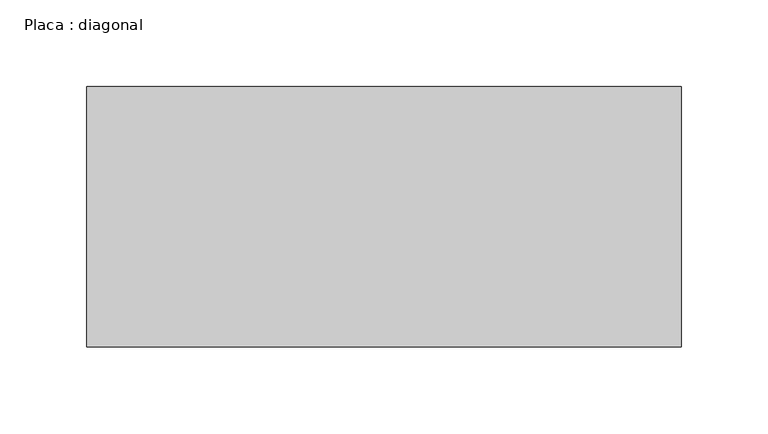
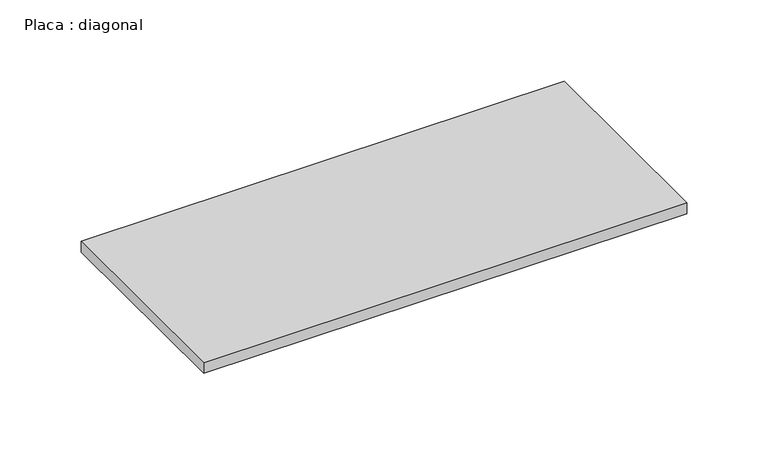
"""IFC4 building model written with IfcOpenShell, lengths in millimetres: beam geometry, Placa : diagonal."""

from ifc_helpers import new_model, si_unit, frame, origin, place, context, project, spatial, polyline, outline, extrude, source, transform, mapped, element, save


def placa_diagonal_34e101ca(model_context):
    return source(origin(), model_context, "Body", "SweptSolid", [
        extrude(outline(polyline([(171.6122421, 75.0), (171.6122421, -75.0), (-170.6977789, -75.0), (-170.6977789, 75.0), (171.6122421, 75.0)])), frame((0.0, 0.0, -4.0), z_axis=(0.0, 0.0, 1.0), x_axis=(1.0, 0.0, 0.0)), (0.0, 0.0, 1.0), 8.0),
    ])


if __name__ == "__main__":
    model = new_model("IFC4")
    model_context = context("Model", 3, world=origin())
    ifc_project = project(units=[si_unit("LENGTHUNIT", "METRE", prefix="MILLI")], contexts=[model_context])
    site = spatial("IfcSite", under=ifc_project)
    building = spatial("IfcBuilding", under=site)
    placement = place(None, origin())
    placa_diagonal_shape = placa_diagonal_34e101ca(model_context)
    element("IfcBeam", 1, ObjectType="Placa : diagonal", at=placement, inside=building, context=model_context, shape_type="MappedRepresentation", body=[
        mapped(placa_diagonal_shape, transform((0.0, 0.0, 0.0), x_axis=(1.0, 0.0, 0.0), y_axis=(0.0, 1.0, 0.0), z_axis=(0.0, 0.0, 1.0))),
    ])
    save(model, "model.ifc")

# Revit data of these elements
# Type "Placa : diagonal"
#   W = 0
#   Length [instance default] = 1.50 m
#   b = 0.15 m
#   d = 0.008 m
#   A = 0 m²
#   Structural Material [instance default] = Aço, 45-345
# Element 1 (IfcBeam, "Placa : diagonal")
#   Materials on its faces: "Aço, 45-345"
# Materials
#   "Aço, 45-345": class "Metal", colour RGB 247 247 247, transparency 0, Description = "Aço 345 MPa", Cost = 0
